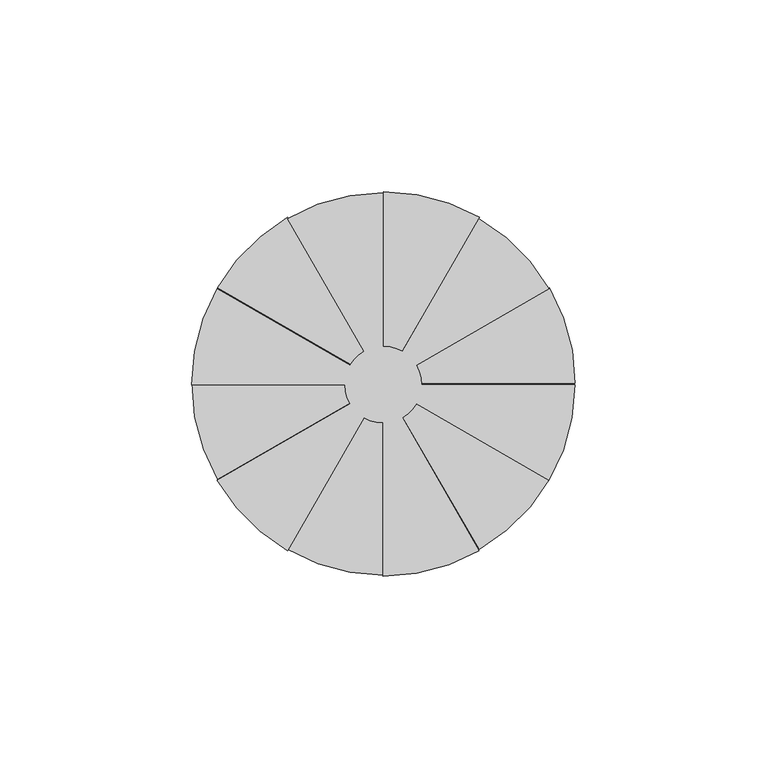
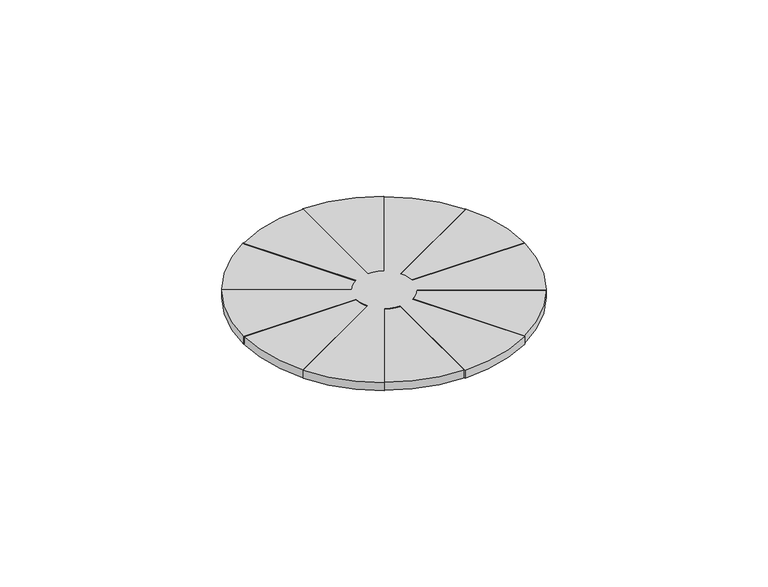
"""IFC4 building model written with IfcOpenShell, lengths in millimetres: proxy geometry, TSP Bathroom Extractor Point-Wall : TSP Bathroom Extractor Point-Wall."""

from ifc_helpers import new_model, si_unit, point, frame_2d, origin, origin_with_axes, place, context, project, spatial, polyline, circle_curve, trimmed, segment, composite_curve, outline, extrude, source, transform, mapped, element, save


def electrical_fixtures_6b2912d0(model_context):
    return source(origin(), model_context, "Body", "SweptSolid", [
        extrude(outline(composite_curve([segment(trimmed(circle_curve(frame_2d((-50.0, 0.0)), 50.0), [point((-100.0, 0.0))], [point((-93.3012702, 25.0))], False, "CARTESIAN"), True, "CONTINUOUS"), segment(polyline([(-93.3012702, 25.0), (-58.660254, 5.0)]), True, "CONTINUOUS"), segment(trimmed(circle_curve(frame_2d((-50.0, 0.0)), 10.0), [point((-58.660254, 5.0))], [point((-55.0, 8.660254))], False, "CARTESIAN"), True, "CONTINUOUS"), segment(polyline([(-55.0, 8.660254), (-75.0, 43.3012702)]), True, "CONTINUOUS"), segment(trimmed(circle_curve(frame_2d((-50.0, 0.0)), 50.0), [point((-75.0, 43.3012702))], [point((-50.0, 50.0))], False, "CARTESIAN"), True, "CONTINUOUS"), segment(polyline([(-50.0, 50.0), (-50.0, 10.0)]), True, "CONTINUOUS"), segment(trimmed(circle_curve(frame_2d((-50.0, 0.0)), 10.0), [point((-50.0, 10.0))], [point((-45.0, 8.660254))], False, "CARTESIAN"), True, "CONTINUOUS"), segment(polyline([(-45.0, 8.660254), (-25.0, 43.3012702)]), True, "CONTINUOUS"), segment(trimmed(circle_curve(frame_2d((-50.0, 0.0)), 50.0), [point((-25.0, 43.3012702))], [point((-6.6987298, 25.0))], False, "CARTESIAN"), True, "CONTINUOUS"), segment(polyline([(-6.6987298, 25.0), (-41.339746, 5.0)]), True, "CONTINUOUS"), segment(trimmed(circle_curve(frame_2d((-50.0, 0.0)), 10.0), [point((-41.339746, 5.0))], [point((-40.0, 0.0))], False, "CARTESIAN"), True, "CONTINUOUS"), segment(polyline([(-40.0, 0.0), (0.0, 0.0)]), True, "CONTINUOUS"), segment(trimmed(circle_curve(frame_2d((-50.0, 0.0)), 50.0), [point((0.0, 0.0))], [point((-6.6987298, -25.0))], False, "CARTESIAN"), True, "CONTINUOUS"), segment(polyline([(-6.6987298, -25.0), (-41.339746, -5.0)]), True, "CONTINUOUS"), segment(trimmed(circle_curve(frame_2d((-50.0, 0.0)), 10.0), [point((-41.339746, -5.0))], [point((-45.0, -8.660254))], False, "CARTESIAN"), True, "CONTINUOUS"), segment(polyline([(-45.0, -8.660254), (-25.0, -43.3012702)]), True, "CONTINUOUS"), segment(trimmed(circle_curve(frame_2d((-50.0, 0.0)), 50.0), [point((-25.0, -43.3012702))], [point((-50.0, -50.0))], False, "CARTESIAN"), True, "CONTINUOUS"), segment(polyline([(-50.0, -50.0), (-50.0, -10.0)]), True, "CONTINUOUS"), segment(trimmed(circle_curve(frame_2d((-50.0, 0.0)), 10.0), [point((-50.0, -10.0))], [point((-55.0, -8.660254))], False, "CARTESIAN"), True, "CONTINUOUS"), segment(polyline([(-55.0, -8.660254), (-75.0, -43.3012702)]), True, "CONTINUOUS"), segment(trimmed(circle_curve(frame_2d((-50.0, 0.0)), 50.0), [point((-75.0, -43.3012702))], [point((-93.3012702, -25.0))], False, "CARTESIAN"), True, "CONTINUOUS"), segment(polyline([(-93.3012702, -25.0), (-58.660254, -5.0)]), True, "CONTINUOUS"), segment(trimmed(circle_curve(frame_2d((-50.0, 0.0)), 10.0), [point((-58.660254, -5.0))], [point((-60.0, 0.0))], False, "CARTESIAN"), True, "CONTINUOUS"), segment(polyline([(-60.0, 0.0), (-100.0, 0.0)]), True, "CONTINUOUS")], self_intersect=False)), origin_with_axes(), (0.0, 0.0, 1.0), 3.0),
        extrude(outline(composite_curve([segment(trimmed(circle_curve(frame_2d((-49.921082, 0.2945262)), 50.0), [point((-93.2223521, 25.2945262))], [point((-74.921082, 43.5957963))], False, "CARTESIAN"), True, "CONTINUOUS"), segment(polyline([(-74.921082, 43.5957963), (-54.921082, 8.9547802)]), True, "CONTINUOUS"), segment(trimmed(circle_curve(frame_2d((-49.921082, 0.2945262)), 10.0), [point((-54.921082, 8.9547802))], [point((-49.921082, 10.2945262))], False, "CARTESIAN"), True, "CONTINUOUS"), segment(polyline([(-49.921082, 10.2945262), (-49.921082, 50.2945262)]), True, "CONTINUOUS"), segment(trimmed(circle_curve(frame_2d((-49.921082, 0.2945262)), 50.0), [point((-49.921082, 50.2945262))], [point((-24.921082, 43.5957963))], False, "CARTESIAN"), True, "CONTINUOUS"), segment(polyline([(-24.921082, 43.5957963), (-44.921082, 8.9547802)]), True, "CONTINUOUS"), segment(trimmed(circle_curve(frame_2d((-49.921082, 0.2945262)), 10.0), [point((-44.921082, 8.9547802))], [point((-41.2608279, 5.2945262))], False, "CARTESIAN"), True, "CONTINUOUS"), segment(polyline([(-41.2608279, 5.2945262), (-6.6198118, 25.2945262)]), True, "CONTINUOUS"), segment(trimmed(circle_curve(frame_2d((-49.921082, 0.2945262)), 50.0), [point((-6.6198118, 25.2945262))], [point((0.078918, 0.2945262))], False, "CARTESIAN"), True, "CONTINUOUS"), segment(polyline([(0.078918, 0.2945262), (-39.921082, 0.2945262)]), True, "CONTINUOUS"), segment(trimmed(circle_curve(frame_2d((-49.921082, 0.2945262)), 10.0), [point((-39.921082, 0.2945262))], [point((-41.2608279, -4.7054738))], False, "CARTESIAN"), True, "CONTINUOUS"), segment(polyline([(-41.2608279, -4.7054738), (-6.6198118, -24.7054738)]), True, "CONTINUOUS"), segment(trimmed(circle_curve(frame_2d((-49.921082, 0.2945262)), 50.0), [point((-6.6198118, -24.7054738))], [point((-24.921082, -43.006744))], False, "CARTESIAN"), True, "CONTINUOUS"), segment(polyline([(-24.921082, -43.006744), (-44.921082, -8.3657279)]), True, "CONTINUOUS"), segment(trimmed(circle_curve(frame_2d((-49.921082, 0.2945262)), 10.0), [point((-44.921082, -8.3657279))], [point((-49.921082, -9.7054738))], False, "CARTESIAN"), True, "CONTINUOUS"), segment(polyline([(-49.921082, -9.7054738), (-49.921082, -49.7054738)]), True, "CONTINUOUS"), segment(trimmed(circle_curve(frame_2d((-49.921082, 0.2945262)), 50.0), [point((-49.921082, -49.7054738))], [point((-74.921082, -43.006744))], False, "CARTESIAN"), True, "CONTINUOUS"), segment(polyline([(-74.921082, -43.006744), (-54.921082, -8.3657279)]), True, "CONTINUOUS"), segment(trimmed(circle_curve(frame_2d((-49.921082, 0.2945262)), 10.0), [point((-54.921082, -8.3657279))], [point((-58.581336, -4.7054738))], False, "CARTESIAN"), True, "CONTINUOUS"), segment(polyline([(-58.581336, -4.7054738), (-93.2223521, -24.7054738)]), True, "CONTINUOUS"), segment(trimmed(circle_curve(frame_2d((-49.921082, 0.2945262)), 50.0), [point((-93.2223521, -24.7054738))], [point((-99.921082, 0.2945262))], False, "CARTESIAN"), True, "CONTINUOUS"), segment(polyline([(-99.921082, 0.2945262), (-59.921082, 0.2945262)]), True, "CONTINUOUS"), segment(trimmed(circle_curve(frame_2d((-49.921082, 0.2945262)), 10.0), [point((-59.921082, 0.2945262))], [point((-58.581336, 5.2945262))], False, "CARTESIAN"), True, "CONTINUOUS"), segment(polyline([(-58.581336, 5.2945262), (-93.2223521, 25.2945262)]), True, "CONTINUOUS")], self_intersect=False)), origin_with_axes(), (0.0, 0.0, 1.0), 3.0),
    ])


if __name__ == "__main__":
    model = new_model("IFC4")
    model_context = context("Model", 3, world=origin())
    ifc_project = project(units=[si_unit("LENGTHUNIT", "METRE", prefix="MILLI")], contexts=[model_context])
    site = spatial("IfcSite", under=ifc_project)
    building = spatial("IfcBuilding", under=site)
    placement = place(None, origin())
    electrical_fixtures_shape = electrical_fixtures_6b2912d0(model_context)
    element("IfcBuildingElementProxy", 1, Name="TSP Bathroom Extractor Point-Wall : TSP Bathroom Extractor Point-Wall", ObjectType="TSP Bathroom Extractor Point-Wall : TSP Bathroom Extractor Point-Wall", at=placement, inside=building, context=model_context, shape_type="MappedRepresentation", body=[
        mapped(electrical_fixtures_shape, transform((0.0, 0.0, 0.0), x_axis=(1.0, 0.0, 0.0), y_axis=(0.0, 1.0, 0.0), z_axis=(0.0, 0.0, 1.0))),
    ])
    save(model, "model.ifc")

# Revit data of these elements
# Type "TSP Bathroom Extractor Point-Wall : TSP Bathroom Extractor Point-Wall"
#   Model = "TSP_ELECBEFPW"
#   Default Elevation = 0
# Element 1 (IfcBuildingElementProxy, "TSP Bathroom Extractor Point-Wall : TSP Bathroom Extractor Point-Wall")
#   Materials on its faces: "Plastic, Opaque Black", "Aluminum, Anodized Blue"
# Materials
#   "Plastic, Opaque Black": class "Plastic", colour RGB 0 0 0, transparency 0.7, Description = "Plastic, generic, opaque black", Cost = 0
#   "Aluminum, Anodized Blue": class "Metal", colour RGB 120 120 120, transparency 0, Description = "Anodized aluminum, blue", Cost = 0
